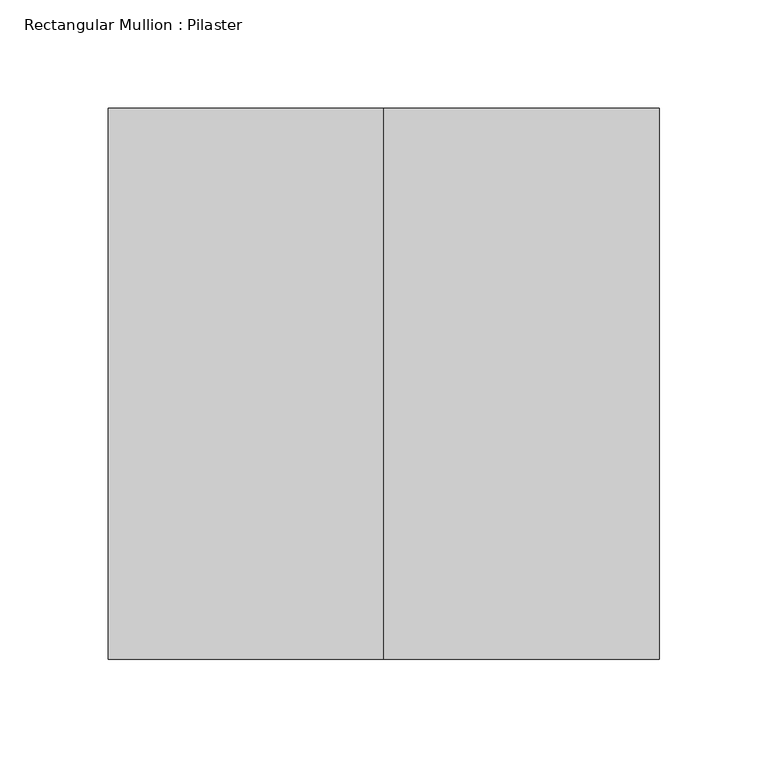
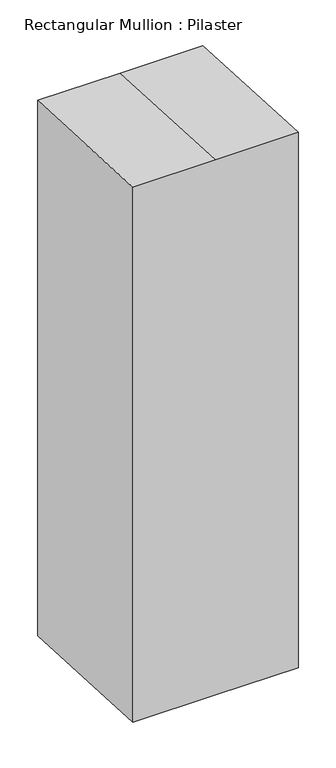
"""IFC4 building model written with IfcOpenShell, lengths in millimetres: member geometry, Rectangular Mullion : Pilaster."""

import ifcopenshell
import ifcopenshell.guid

model = None  # the IFC model being written
_history = None  # IfcOwnerHistory: only IFC2X3 demands one
_inside = {}  # id of a spatial element -> (the spatial element, [elements in it])
_under = {}  # id of a project, library or spatial element -> (it, [spatial elements below it])
_declared = {}  # id of a project -> (the project, [libraries it declares])
_typed = {}  # id of a type object -> (the type object, [elements of that type])
_made_of = {}  # id of a material, layer set ... -> (it, [elements and type objects made of it])


def new_model(schema):
    """Start an empty IFC model of exactly this schema.

    Asked for "IFC4X3", IfcOpenShell would pick the latest addendum, in which some entities
    have other attributes; the version numbers below select the first issue.
    IFC2X3 requires an IfcOwnerHistory on every rooted entity: one is made here for all.
    """
    global model, _history
    if schema == "IFC4X3":
        model = ifcopenshell.file(schema_version=(4, 3, 0, 0))
    else:
        model = ifcopenshell.file(schema=schema)
    _inside.clear()
    _under.clear()
    _declared.clear()
    _typed.clear()
    _made_of.clear()
    _history = None
    if model.schema == "IFC2X3":
        org = make("IfcOrganization", Name="unknown")
        user = make(
            "IfcPersonAndOrganization",
            ThePerson=make("IfcPerson", FamilyName="unknown"),
            TheOrganization=org,
        )
        app = make(
            "IfcApplication",
            ApplicationDeveloper=org,
            Version="unknown",
            ApplicationFullName="unknown",
            ApplicationIdentifier="unknown",
        )
        _history = make(
            "IfcOwnerHistory",
            OwningUser=user,
            OwningApplication=app,
            ChangeAction="ADDED",
            CreationDate=0,
        )
    return model


def make(cls, **values):
    """One entity of the class cls with the attributes given. An attribute that is None is left unset."""
    return model.create_entity(
        cls, **{name: value for name, value in values.items() if value is not None}
    )


def rooted(cls, **values):
    """An entity with a GlobalId (a new one), such as an element, a storey or a relation."""
    return make(cls, GlobalId=ifcopenshell.guid.new(), OwnerHistory=_history, **values)


def si_unit(unit_type, name, prefix=None):
    """IfcSIUnit, for example si_unit("LENGTHUNIT", "METRE", prefix="MILLI")."""
    return make("IfcSIUnit", UnitType=unit_type, Prefix=prefix, Name=name)


def assignment(units):
    """IfcUnitAssignment: the units of a project."""
    return None if units is None else make("IfcUnitAssignment", Units=units)


def point(xyz):
    """IfcCartesianPoint."""
    return None if xyz is None else make("IfcCartesianPoint", Coordinates=xyz)


def direction(xyz):
    """IfcDirection."""
    return None if xyz is None else make("IfcDirection", DirectionRatios=xyz)


def frame(location, z_axis=None, x_axis=None):
    """IfcAxis2Placement3D, a coordinate frame: its origin and axes. An axis left out is left unset."""
    return make(
        "IfcAxis2Placement3D",
        Location=point(location),
        Axis=direction(z_axis),
        RefDirection=direction(x_axis),
    )


def origin():
    """The frame at (0, 0, 0) with its axes left unset."""
    return frame((0.0, 0.0, 0.0))


def place(relative_to, where):
    """IfcLocalPlacement: puts the frame where relative to a parent placement (None: the world)."""
    return make(
        "IfcLocalPlacement", PlacementRelTo=relative_to, RelativePlacement=where
    )


def context(
    kind, dimensions, precision=None, world=None, true_north=None, identifier=None
):
    """IfcGeometricRepresentationContext, for example the 3D "Model" context."""
    return make(
        "IfcGeometricRepresentationContext",
        ContextIdentifier=identifier,
        ContextType=kind,
        CoordinateSpaceDimension=dimensions,
        Precision=precision,
        WorldCoordinateSystem=world,
        TrueNorth=true_north,
    )


def project(units=None, contexts=None):
    """IfcProject with its units and contexts."""
    return rooted(
        "IfcProject",
        Name="project",
        RepresentationContexts=contexts,
        UnitsInContext=assignment(units),
    )


def spatial(cls, under=None, at=None, **own):
    """A site, building, storey or space (cls), placed at a placement, below another one or the project."""
    s = rooted(cls, ObjectPlacement=at, **own)
    if under is not None:
        _under.setdefault(under.id(), (under, []))[1].append(s)
    return s


def faces_of(points, faces, orient=None, outer=None):
    """IfcFace entities. A face is a list of loops; a loop is a list of indices into points, from 0.

    orient and outer hold one flag for each loop. By default every Orientation is true, the
    first loop of a face is its IfcFaceOuterBound and the others are IfcFaceBound.
    """
    made = []
    for i, loops in enumerate(faces):
        bounds = []
        for j, loop in enumerate(loops):
            is_outer = j == 0 if outer is None else outer[i][j]
            bounds.append(
                make(
                    "IfcFaceOuterBound" if is_outer else "IfcFaceBound",
                    Bound=make("IfcPolyLoop", Polygon=[points[k] for k in loop]),
                    Orientation=True if orient is None else orient[i][j],
                )
            )
        made.append(make("IfcFace", Bounds=bounds))
    return made


def faceted_brep(points, faces, orient=None, outer=None, voids=None):
    """IfcFacetedBrep: a solid bounded by flat faces; with voids (closed shells), ...WithVoids."""
    shared = [point(p) for p in points]
    hull = make("IfcClosedShell", CfsFaces=faces_of(shared, faces, orient, outer))
    if voids is None:
        return make("IfcFacetedBrep", Outer=hull)
    return make(
        "IfcFacetedBrepWithVoids",
        Outer=hull,
        Voids=[
            make(cls, CfsFaces=faces_of(shared, fs, o, b)) for cls, fs, o, b in voids
        ],
    )


def shape(context_of_items, identifier, shape_type, items):
    """IfcShapeRepresentation: the items that make up one representation, for example the "Body"."""
    return make(
        "IfcShapeRepresentation",
        ContextOfItems=context_of_items,
        RepresentationIdentifier=identifier,
        RepresentationType=shape_type,
        Items=items,
    )


def source(mapping_origin, context_of_items, identifier, shape_type, items):
    """IfcRepresentationMap: a shape defined once, which mapped items show again and again."""
    return make(
        "IfcRepresentationMap",
        MappingOrigin=mapping_origin,
        MappedRepresentation=shape(context_of_items, identifier, shape_type, items),
    )


def transform(
    local_origin,
    x_axis=None,
    y_axis=None,
    z_axis=None,
    scale=None,
    scale2=None,
    scale3=None,
    uniform=True,
):
    """IfcCartesianTransformationOperator3D, or its non-uniform kind. x_axis, y_axis, z_axis: its Axis1, 2, 3."""
    if uniform:
        return make(
            "IfcCartesianTransformationOperator3D",
            Axis1=direction(x_axis),
            Axis2=direction(y_axis),
            LocalOrigin=point(local_origin),
            Scale=scale,
            Axis3=direction(z_axis),
        )
    return make(
        "IfcCartesianTransformationOperator3DnonUniform",
        Axis1=direction(x_axis),
        Axis2=direction(y_axis),
        LocalOrigin=point(local_origin),
        Scale=scale,
        Axis3=direction(z_axis),
        Scale2=scale2,
        Scale3=scale3,
    )


def mapped(mapping_source, mapping_target):
    """IfcMappedItem: shows the shape of a source again, moved by a transform."""
    return make(
        "IfcMappedItem", MappingSource=mapping_source, MappingTarget=mapping_target
    )


def made_of(thing, what):
    """Note that an element or type object is made of a material, layer set ...; save() writes the relation."""
    if what is not None:
        _made_of.setdefault(what.id(), (what, []))[1].append(thing)
    return thing


def element(
    cls,
    number,
    at=None,
    inside=None,
    cuts=None,
    type_object=None,
    material=None,
    context=None,
    identifier="Body",
    shape_type=None,
    held_by="IfcProductDefinitionShape",
    body=None,
    shapes=None,
    **own,
):
    """One element of the class cls, such as IfcWall. Its Tag is "e" and its number.

    at: its placement. inside: the storey or other place that contains it. cuts: it is an
    opening in that element (IfcRelVoidsElement). A single representation is given by context,
    identifier, shape_type and body (its items); several are given by shapes. held_by: the class
    of the entity that holds the representations. save() writes the other relations.
    """
    e = rooted(cls, Tag="e%d" % number, ObjectPlacement=at, **own)
    if body is not None:
        shapes = [shape(context, identifier, shape_type, body)]
    if shapes is not None:
        e.Representation = make(held_by, Representations=shapes)
    if inside is not None:
        _inside.setdefault(inside.id(), (inside, []))[1].append(e)
    if cuts is not None:
        rooted(
            "IfcRelVoidsElement", RelatingBuildingElement=cuts, RelatedOpeningElement=e
        )
    if type_object is not None:
        _typed.setdefault(type_object.id(), (type_object, []))[1].append(e)
    return made_of(e, material)


def aggregate(whole, parts):
    """IfcRelAggregates: a whole, such as a stair, and the parts it consists of."""
    return rooted("IfcRelAggregates", RelatingObject=whole, RelatedObjects=parts)


def save(model, path):
    """Write the relations noted so far, then the file.

    IfcRelAggregates (storeys below a building ...), IfcRelContainedInSpatialStructure (elements
    in a storey), IfcRelDefinesByType, IfcRelAssociatesMaterial and IfcRelDeclares: one each for
    every whole, place, type object, material and project.
    """
    for whole, parts in _under.values():
        aggregate(whole, parts)
    for where, things in _inside.values():
        rooted(
            "IfcRelContainedInSpatialStructure",
            RelatedElements=things,
            RelatingStructure=where,
        )
    for kind, things in _typed.values():
        rooted("IfcRelDefinesByType", RelatedObjects=things, RelatingType=kind)
    for what, things in _made_of.values():
        rooted("IfcRelAssociatesMaterial", RelatedObjects=things, RelatingMaterial=what)
    for by, libraries in _declared.values():
        rooted("IfcRelDeclares", RelatingContext=by, RelatedDefinitions=libraries)
    model.write(path)


def rectangular_mullion_pilaster_fddbf53e(model_context):
    return source(origin(), model_context, "Body", "Brep", [
        faceted_brep([(-127.0, 127.0, -2.7320304), (0.0, 127.0, -2.7320304), (127.0, 127.0, -2.7320304), (127.0, 127.0, -872.2393518), (0.0, 127.0, -872.2393518), (-127.0, 127.0, -872.2393518), (-127.0, -127.0, 10.5795456), (-127.0, -127.0, -858.9277759), (127.0, -127.0, 10.5795456), (0.0, -127.0, 10.5795456), (0.0, -127.0, -858.9277759), (127.0, -127.0, -858.9277759)], [[[0, 1, 2, 3, 4, 5]], [[6, 0, 5, 7]], [[8, 9, 6, 7, 10, 11]], [[2, 8, 11, 3]], [[2, 1, 9, 8]], [[1, 0, 6, 9]], [[3, 11, 10, 4]], [[10, 7, 5, 4]]]),
    ])


if __name__ == "__main__":
    model = new_model("IFC4")
    model_context = context("Model", 3, world=origin())
    ifc_project = project(units=[si_unit("LENGTHUNIT", "METRE", prefix="MILLI")], contexts=[model_context])
    site = spatial("IfcSite", under=ifc_project)
    building = spatial("IfcBuilding", under=site)
    placement = place(None, origin())
    rectangular_mullion_pilaster_shape = rectangular_mullion_pilaster_fddbf53e(model_context)
    element("IfcMember", 1, ObjectType="Rectangular Mullion : Pilaster", at=placement, inside=building, context=model_context, shape_type="MappedRepresentation", body=[
        mapped(rectangular_mullion_pilaster_shape, transform((0.0, 0.0, 0.0), x_axis=(1.0, 0.0, 0.0), y_axis=(0.0, 1.0, 0.0), z_axis=(0.0, 0.0, 1.0))),
    ])
    save(model, "model.ifc")

# Revit data of these elements
# Type "Rectangular Mullion : Pilaster"
#   built-in parameter 1007304 = 0.833333 (stored number, unit not read)
#   built-in parameter 1007301 = 0.416667 (stored number, unit not read)
#   built-in parameter 1007300 = 0.416667 (stored number, unit not read)
# Element 1 (IfcMember, "Rectangular Mullion : Pilaster")
#   Materials on its faces: "Aluminum"
# Materials
#   "Aluminum": class "Metal", colour RGB 247 247 247, transparency 0, Description = "Aluminum 6061", Cost = 0
